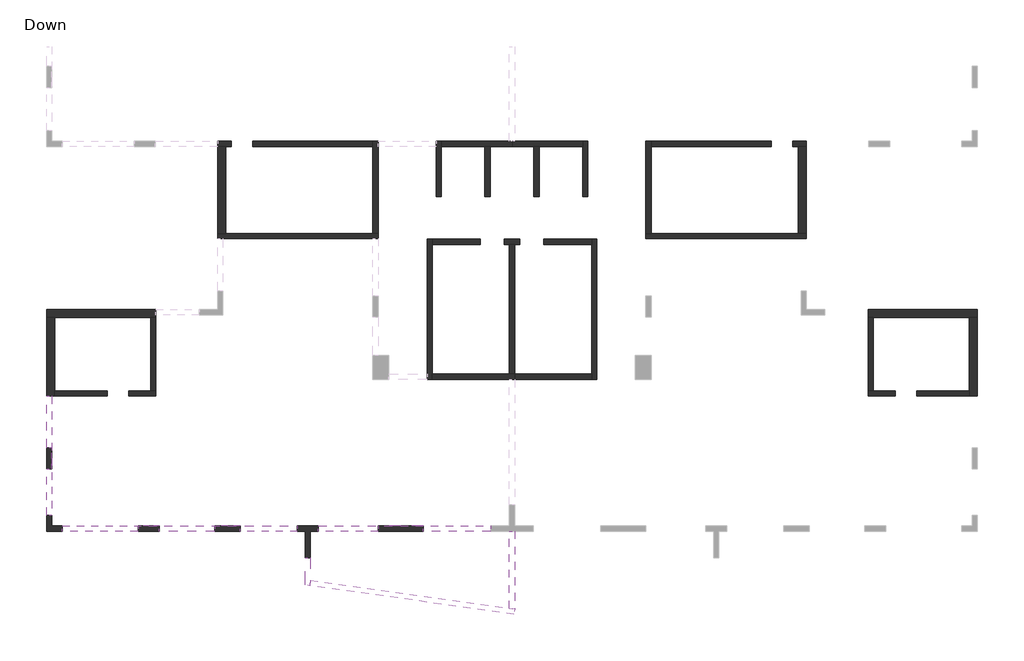
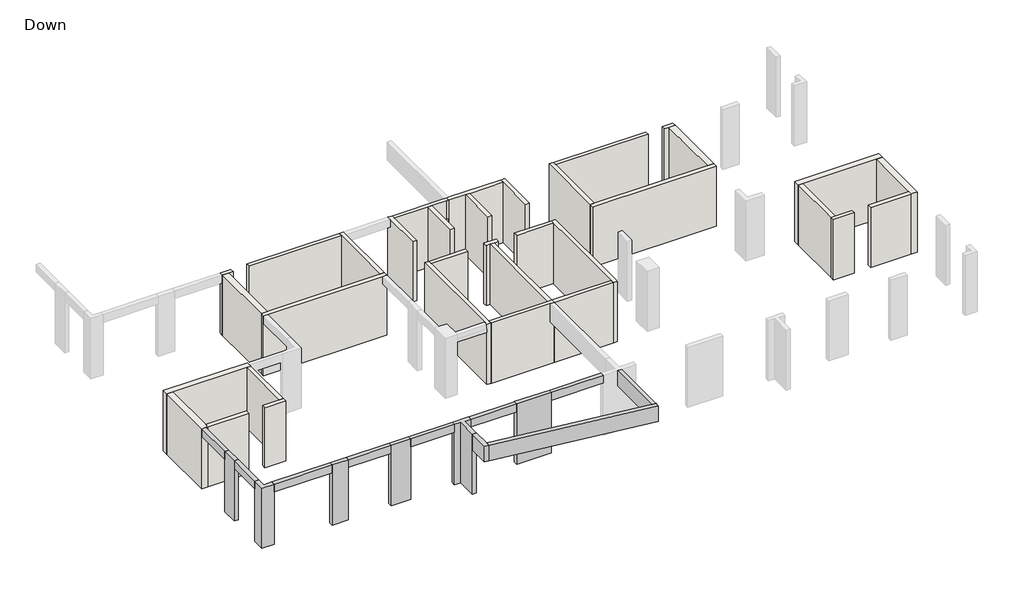
# One storey, part 1 of 2: 34 walls, 10 beams, 6 columns.
"""IFC4 building model written with IfcOpenShell, lengths in millimetres."""

from ifc_helpers import new_model, si_unit, origin, origin_with_axes, place, context, project, spatial, polyline, outline, extrude, faceted_brep, element, save

model = new_model("IFC4")

# Units and contexts
model_context = context("Model", 3, world=origin())
ifc_project = project(units=[si_unit("LENGTHUNIT", "METRE", prefix="MILLI")], contexts=[model_context])

# Site, building, storey
site = spatial("IfcSite", under=ifc_project)
building = spatial("IfcBuilding", under=site)
storey = spatial("IfcBuildingStorey", under=building, Name="Down", Elevation=0.0)

# Beams
placement = place(None, origin())
element("IfcBeam", 1, ObjectType="Concrete Rectengular Beam : 20/40", at=placement, inside=storey, context=model_context, shape_type="Brep", body=[
    faceted_brep([(-5966.3203921, -13204.5252202, 3120.0), (-3416.392751, -13204.5252202, 3120.0), (-3416.392751, -13009.5252202, 3120.0), (-5966.3203921, -13009.5252202, 3120.0), (-3416.392751, -13004.5252202, 2720.0), (-6816.392751, -13004.5252202, 2720.0), (-6816.392751, -13004.5252202, 2890.0), (-3416.392751, -13004.5252202, 2890.0), (-3416.392751, -13204.5252202, 2720.0), (-5966.3203921, -13204.5252202, 2720.0), (-5966.3203921, -13005.5744243, 2720.0), (-6816.392751, -13005.5744243, 2720.0), (-5966.3203921, -13204.5252202, 2890.0), (-6816.392751, -13005.5744243, 2890.0), (-3416.392751, -13009.5252202, 2890.0), (-5966.3203921, -13005.5744243, 2890.0), (-5966.3203921, -13009.5252202, 2890.0)], [[[0, 1, 2, 3]], [[4, 5, 6, 7]], [[5, 4, 8, 9, 10, 11]], [[8, 1, 0, 12, 9]], [[5, 11, 13, 6]], [[8, 4, 7, 14, 2, 1]], [[11, 10, 15, 13]], [[10, 9, 12, 0, 3, 16, 15]], [[16, 14, 7, 6, 13, 15]], [[14, 16, 3, 2]]]),
])
element("IfcBeam", 2, ObjectType="Concrete Rectengular Beam : 20/40", at=placement, inside=storey, context=model_context, shape_type="Brep", body=[
    faceted_brep([(-7666.3203921, -13204.5252202, 3120.0), (-7666.3203921, -13009.5252202, 3120.0), (-9916.193764, -13009.5252202, 3120.0), (-9916.193764, -13204.5252202, 3120.0), (-6816.392751, -13004.5252202, 2890.0), (-6816.392751, -13004.5252202, 2720.0), (-9916.193764, -13004.5252202, 2720.0), (-9916.193764, -13004.5252202, 2890.0), (-6816.392751, -13005.5744243, 2720.0), (-7666.3203921, -13005.5744243, 2720.0), (-7666.3203921, -13204.5252202, 2720.0), (-9916.193764, -13204.5252202, 2720.0), (-7666.3203921, -13204.5252202, 2890.0), (-6816.392751, -13005.5744243, 2890.0), (-7666.3203921, -13005.5744243, 2890.0), (-7666.3203921, -13009.5252202, 2890.0), (-9916.193764, -13009.5252202, 2890.0)], [[[0, 1, 2, 3]], [[4, 5, 6, 7]], [[5, 8, 9, 10, 11, 6]], [[10, 12, 0, 3, 11]], [[8, 5, 4, 13]], [[9, 8, 13, 14]], [[10, 9, 14, 15, 1, 0, 12]], [[13, 4, 7, 16, 15, 14]], [[1, 15, 16, 2]], [[3, 2, 16, 7, 6, 11]]]),
])
element("IfcBeam", 3, ObjectType="Concrete Rectengular Beam : 20/40", at=placement, inside=storey, context=model_context, shape_type="Brep", body=[
    faceted_brep([(-12866.5555585, -13009.5252202, 3120.0), (-12866.5555585, -13204.5252202, 3120.0), (-10716.193764, -13204.5252202, 3120.0), (-10716.193764, -13009.5252202, 3120.0), (-13341.5555585, -13004.5252202, 2720.0), (-13341.5555585, -13004.5252202, 2890.0), (-10716.193764, -13004.5252202, 2890.0), (-10716.193764, -13004.5252202, 2720.0), (-13341.5555585, -13005.8747137, 2720.0), (-10716.193764, -13204.5252202, 2720.0), (-12866.5555585, -13204.5252202, 2720.0), (-12866.5555585, -13005.8747137, 2720.0), (-13341.5555585, -13005.8747137, 2890.0), (-12866.5555585, -13005.8747137, 2890.0), (-12866.5555585, -13009.5252202, 2890.0), (-10716.193764, -13009.5252202, 2890.0)], [[[0, 1, 2, 3]], [[4, 5, 6, 7]], [[8, 4, 7, 9, 10, 11]], [[1, 10, 9, 2]], [[4, 8, 12, 5]], [[8, 11, 13, 12]], [[11, 10, 1, 0, 14, 13]], [[5, 12, 13, 14, 15, 6]], [[14, 0, 3, 15]], [[3, 2, 9, 7, 6, 15]]]),
])
element("IfcBeam", 4, ObjectType="Concrete Rectengular Beam : 20/40", at=placement, inside=storey, context=model_context, shape_type="Brep", body=[
    faceted_brep([(-15916.4289304, -13204.5252202, 3120.0), (-13816.5555585, -13204.5252202, 3120.0), (-13816.5555585, -13009.5252202, 3120.0), (-15916.4289304, -13009.5252202, 3120.0), (-13341.5555585, -13004.5252202, 2720.0), (-16316.4289304, -13004.5252202, 2720.0), (-16316.4289304, -13004.5252202, 2890.0), (-13341.5555585, -13004.5252202, 2890.0), (-13341.5555585, -13005.8747137, 2720.0), (-13816.5555585, -13005.8747137, 2720.0), (-13816.5555585, -13204.5252202, 2720.0), (-15916.4289304, -13204.5252202, 2720.0), (-15916.4289304, -13005.8747137, 2720.0), (-16316.4289304, -13005.8747137, 2720.0), (-16316.4289304, -13005.8747137, 2890.0), (-13341.5555585, -13005.8747137, 2890.0), (-15916.4289304, -13005.8747137, 2890.0), (-15916.4289304, -13009.5252202, 2890.0), (-13816.5555585, -13005.8747137, 2890.0), (-13816.5555585, -13009.5252202, 2890.0)], [[[0, 1, 2, 3]], [[4, 5, 6, 7]], [[5, 4, 8, 9, 10, 11, 12, 13]], [[0, 11, 10, 1]], [[5, 13, 14, 6]], [[8, 4, 7, 15]], [[13, 12, 16, 14]], [[12, 11, 0, 3, 17, 16]], [[9, 8, 15, 18]], [[10, 9, 18, 19, 2, 1]], [[17, 19, 18, 15, 7, 6, 14, 16]], [[19, 17, 3, 2]]]),
])
element("IfcBeam", 5, ObjectType="Concrete Rectengular Beam : 20/40", at=placement, inside=storey, context=model_context, shape_type="Brep", body=[
    faceted_brep([(-19564.2400737, -13204.5252202, 3120.0), (-16716.4289304, -13204.5252202, 3120.0), (-16716.4289304, -13009.5252202, 3120.0), (-19564.2400737, -13009.5252202, 3120.0), (-16316.4289304, -13004.5252202, 2720.0), (-19564.2400737, -13004.5252202, 2720.0), (-19564.2400737, -13004.5252202, 2890.0), (-16316.4289304, -13004.5252202, 2890.0), (-16316.4289304, -13005.8747137, 2720.0), (-16716.4289304, -13005.8747137, 2720.0), (-16716.4289304, -13204.5252202, 2720.0), (-19564.2400737, -13204.5252202, 2720.0), (-16316.4289304, -13005.8747137, 2890.0), (-19564.2400737, -13009.5252202, 2890.0), (-16716.4289304, -13005.8747137, 2890.0), (-16716.4289304, -13009.5252202, 2890.0)], [[[0, 1, 2, 3]], [[4, 5, 6, 7]], [[5, 4, 8, 9, 10, 11]], [[0, 11, 10, 1]], [[8, 4, 7, 12]], [[5, 11, 0, 3, 13, 6]], [[9, 8, 12, 14]], [[10, 9, 14, 15, 2, 1]], [[13, 15, 14, 12, 7, 6]], [[15, 13, 3, 2]]]),
])
element("IfcBeam", 6, ObjectType="Concrete Rectengular Beam : 20/40", at=placement, inside=storey, context=model_context, shape_type="Brep", body=[
    faceted_brep([(-20164.2400737, -10855.1764503, 3120.0), (-20164.2400737, -12604.5252202, 3120.0), (-19966.2400737, -12604.5252202, 3120.0), (-19966.2400737, -10855.1764503, 3120.0), (-19964.2400737, -12604.5252202, 2720.0), (-19964.2400737, -10455.1764503, 2720.0), (-19964.2400737, -10455.1764503, 2890.0), (-19964.2400737, -12604.5252202, 2890.0), (-20164.2400737, -12604.5252202, 2720.0), (-20164.2400737, -10855.1764503, 2720.0), (-19965.2892778, -10855.1764503, 2720.0), (-19965.2892778, -10455.1764503, 2720.0), (-19965.2892778, -10455.1764503, 2890.0), (-19966.2400737, -12604.5252202, 2890.0), (-19965.2892778, -10855.1764503, 2890.0), (-19966.2400737, -10855.1764503, 2890.0)], [[[0, 1, 2, 3]], [[4, 5, 6, 7]], [[5, 4, 8, 9, 10, 11]], [[8, 1, 0, 9]], [[5, 11, 12, 6]], [[8, 4, 7, 13, 2, 1]], [[11, 10, 14, 12]], [[10, 9, 0, 3, 15, 14]], [[15, 13, 7, 6, 12, 14]], [[13, 15, 3, 2]]]),
])
element("IfcBeam", 7, ObjectType="Concrete Rectengular Beam : 20/40", at=placement, inside=storey, context=model_context, shape_type="Brep", body=[
    faceted_brep([(-20164.2400737, -8105.8819496, 3120.0), (-20164.2400737, -10055.1764503, 3120.0), (-19966.2400737, -10055.1764503, 3120.0), (-19966.2400737, -8105.8819496, 3120.0), (-19964.2400737, -10455.1764503, 2720.0), (-19964.2400737, -8105.8819496, 2720.0), (-19964.2400737, -8105.8819496, 2890.0), (-19964.2400737, -10455.1764503, 2890.0), (-19965.2892778, -10455.1764503, 2720.0), (-19965.2892778, -10055.1764503, 2720.0), (-20164.2400737, -10055.1764503, 2720.0), (-20164.2400737, -8105.8819496, 2720.0), (-19965.2892778, -10455.1764503, 2890.0), (-19965.2892778, -10055.1764503, 2890.0), (-19966.2400737, -10055.1764503, 2890.0), (-19966.2400737, -8105.8819496, 2890.0)], [[[0, 1, 2, 3]], [[4, 5, 6, 7]], [[4, 8, 9, 10, 11, 5]], [[10, 1, 0, 11]], [[8, 4, 7, 12]], [[9, 8, 12, 13]], [[10, 9, 13, 14, 2, 1]], [[5, 11, 0, 3, 15, 6]], [[15, 14, 13, 12, 7, 6]], [[14, 15, 3, 2]]]),
])
element("IfcBeam", 8, ObjectType="Concrete Rectengular Beam : 20/80", at=placement, inside=storey, context=model_context, shape_type="Brep", body=[
    faceted_brep([(-10416.193764, -15232.5030981, 3120.0), (-10216.193764, -15260.611265, 3120.0), (-10216.193764, -15058.6457505, 3120.0), (-10216.193764, -14204.5252202, 3120.0), (-10416.193764, -14204.5252202, 3120.0), (-10416.193764, -15232.5030981, 2320.0), (-10416.193764, -14204.5252202, 2320.0), (-10216.193764, -15260.611265, 2320.0), (-10216.193764, -14204.5252202, 2320.0), (-10216.193764, -15058.6457505, 2320.0)], [[[0, 1, 2, 3, 4]], [[5, 0, 4, 6]], [[7, 5, 6, 8, 9]], [[1, 7, 9, 8, 3, 2]], [[4, 3, 8, 6]], [[1, 0, 5, 7]]]),
])
element("IfcBeam", 9, ObjectType="Concrete Rectengular Beam : 20/80", at=placement, inside=storey, context=model_context, shape_type="Brep", body=[
    faceted_brep([(-10216.193764, -15058.6457505, 3120.0), (-10216.193764, -15260.611265, 3120.0), (-2544.2273712, -16338.8358257, 3120.0), (-2541.3191471, -16318.142736, 3120.0), (-2516.392751, -16140.7822119, 3120.0), (-2716.392751, -16112.674045, 3120.0), (-10216.193764, -15260.611265, 2320.0), (-2544.2273712, -16338.8358257, 2320.0), (-10216.193764, -15058.6457505, 2320.0), (-2716.392751, -16112.674045, 2320.0), (-2516.392751, -16140.7822119, 2320.0), (-2541.3191471, -16318.142736, 2320.0), (-10216.193764, -15058.6457505, 2890.0)], [[[0, 1, 2, 3, 4, 5]], [[1, 6, 7, 2]], [[6, 8, 9, 10, 11, 7]], [[4, 10, 9, 8, 12, 0, 5]], [[1, 0, 12, 8, 6]], [[4, 3, 2, 7, 11, 10]]]),
])
element("IfcBeam", 10, ObjectType="Concrete Rectengular Beam : 20/80", at=placement, inside=storey, context=model_context, shape_type="Brep", body=[
    faceted_brep([(-2516.392751, -13204.5252202, 3120.0), (-2716.392751, -13204.5252202, 3120.0), (-2716.392751, -16112.674045, 3120.0), (-2516.392751, -16140.7822119, 3120.0), (-2516.392751, -16112.674045, 3120.0), (-2516.392751, -13204.5252202, 2320.0), (-2516.392751, -13204.5252202, 2890.0), (-2516.392751, -16140.7822119, 2320.0), (-2516.392751, -16112.674045, 2320.0), (-2716.392751, -13204.5252202, 2320.0), (-2716.392751, -16112.674045, 2320.0), (-2716.392751, -13204.5252202, 2890.0), (-2716.392751, -16112.674045, 2890.0)], [[[0, 1, 2, 3, 4]], [[5, 6, 0, 4, 3, 7, 8]], [[9, 5, 8, 7, 10]], [[1, 11, 9, 10, 12, 2]], [[1, 0, 6, 5, 9, 11]], [[3, 2, 12, 10, 7]]]),
])

# Columns
element("IfcColumn", 11, ObjectType="Concrete Rectengular Column : 170/20", at=placement, inside=storey, context=model_context, shape_type="Brep", body=[
    faceted_brep([(-7666.3203921, -13005.5744243, 0.0), (-5966.3203921, -13005.5744243, 0.0), (-5966.3203921, -13205.5744243, 0.0), (-7666.3203921, -13205.5744243, 0.0), (-7666.3203921, -13005.5744243, 3120.0), (-5966.3203921, -13005.5744243, 3120.0), (-5966.3203921, -13005.5744243, 2890.0), (-7666.3203921, -13005.5744243, 2890.0), (-5966.3203921, -13009.5252202, 3120.0), (-5966.3203921, -13204.5252202, 3120.0), (-5966.3203921, -13205.5744243, 3120.0), (-5966.3203921, -13205.5744243, 2890.0), (-7666.3203921, -13205.5744243, 3120.0), (-7666.3203921, -13205.5744243, 2890.0), (-7666.3203921, -13204.5252202, 3120.0), (-7666.3203921, -13009.5252202, 3120.0)], [[[0, 1, 2, 3]], [[4, 5, 6, 1, 0, 7]], [[5, 8, 9, 10, 11, 2, 1, 6]], [[10, 12, 13, 3, 2, 11]], [[12, 14, 15, 4, 7, 0, 3, 13]], [[4, 15, 14, 12, 10, 9, 8, 5]]]),
])
element("IfcColumn", 12, ObjectType="Concrete Rectengular Column : 80/20", at=placement, inside=storey, context=model_context, shape_type="Brep", body=[
    faceted_brep([(-16716.4289304, -13005.8747137, 0.0), (-15916.4289304, -13005.8747137, 0.0), (-15916.4289304, -13205.8747137, 0.0), (-16716.4289304, -13205.8747137, 0.0), (-16716.4289304, -13005.8747137, 3120.0), (-15916.4289304, -13005.8747137, 3120.0), (-15916.4289304, -13005.8747137, 2890.0), (-16716.4289304, -13005.8747137, 2890.0), (-15916.4289304, -13009.5252202, 3120.0), (-15916.4289304, -13205.8747137, 3120.0), (-16716.4289304, -13205.8747137, 3120.0), (-16716.4289304, -13009.5252202, 3120.0)], [[[0, 1, 2, 3]], [[4, 5, 6, 1, 0, 7]], [[5, 8, 9, 2, 1, 6]], [[9, 10, 3, 2]], [[10, 11, 4, 7, 0, 3]], [[4, 11, 10, 9, 8, 5]]]),
])
element("IfcColumn", 13, ObjectType="Concrete Rectengular Column : 80/20", at=placement, inside=storey, context=model_context, shape_type="Brep", body=[
    faceted_brep([(-19965.2892778, -10055.1764503, 0.0), (-19965.2892778, -10855.1764503, 0.0), (-20165.2892778, -10855.1764503, 0.0), (-20165.2892778, -10055.1764503, 0.0), (-19965.2892778, -10055.1764503, 3120.0), (-19965.2892778, -10855.1764503, 3120.0), (-19965.2892778, -10855.1764503, 2890.0), (-19965.2892778, -10055.1764503, 2890.0), (-19966.2400737, -10855.1764503, 3120.0), (-20165.2892778, -10855.1764503, 3120.0), (-20165.2892778, -10055.1764503, 3120.0), (-19966.2400737, -10055.1764503, 3120.0)], [[[0, 1, 2, 3]], [[4, 5, 6, 1, 0, 7]], [[5, 8, 9, 2, 1, 6]], [[9, 10, 3, 2]], [[10, 11, 4, 7, 0, 3]], [[4, 11, 10, 9, 8, 5]]]),
])
element("IfcColumn", 14, ObjectType="Concrete Rectengular Column : 95/20", at=placement, inside=storey, context=model_context, shape_type="Brep", body=[
    faceted_brep([(-13816.5555585, -13005.8747137, 0.0), (-12866.5555585, -13005.8747137, 0.0), (-12866.5555585, -13205.8747137, 0.0), (-13816.5555585, -13205.8747137, 0.0), (-13816.5555585, -13005.8747137, 3120.0), (-12866.5555585, -13005.8747137, 3120.0), (-12866.5555585, -13005.8747137, 2890.0), (-13816.5555585, -13005.8747137, 2890.0), (-12866.5555585, -13009.5252202, 3120.0), (-12866.5555585, -13205.8747137, 3120.0), (-13816.5555585, -13205.8747137, 3120.0), (-13816.5555585, -13009.5252202, 3120.0)], [[[0, 1, 2, 3]], [[4, 5, 6, 1, 0, 7]], [[5, 8, 9, 2, 1, 6]], [[9, 10, 3, 2]], [[10, 11, 4, 7, 0, 3]], [[4, 11, 10, 9, 8, 5]]]),
])
element("IfcColumn", 15, ObjectType="L Column : 60/60/20/20", at=placement, inside=storey, context=model_context, shape_type="Brep", body=[
    faceted_brep([(-20164.2400737, -13204.5252202, 0.0), (-20164.2400737, -12604.5252202, 0.0), (-19964.2400737, -12604.5252202, 0.0), (-19964.2400737, -13004.5252202, 0.0), (-19564.2400737, -13004.5252202, 0.0), (-19564.2400737, -13204.5252202, 0.0), (-20164.2400737, -13204.5252202, 3120.0), (-20164.2400737, -12604.5252202, 3120.0), (-19966.2400737, -12604.5252202, 3120.0), (-19964.2400737, -12604.5252202, 3120.0), (-19964.2400737, -12604.5252202, 2890.0), (-19964.2400737, -13004.5252202, 3120.0), (-19964.2400737, -13004.5252202, 2890.0), (-19564.2400737, -13004.5252202, 3120.0), (-19564.2400737, -13004.5252202, 2890.0), (-19564.2400737, -13009.5252202, 3120.0), (-19564.2400737, -13204.5252202, 3120.0)], [[[0, 1, 2, 3, 4, 5]], [[6, 7, 1, 0]], [[7, 8, 9, 10, 2, 1]], [[9, 11, 12, 3, 2, 10]], [[11, 13, 14, 4, 3, 12]], [[13, 15, 16, 5, 4, 14]], [[16, 6, 0, 5]], [[6, 16, 15, 13, 11, 9, 8, 7]]]),
])
element("IfcColumn", 16, ObjectType="T Column : 120/80/20/20", at=placement, inside=storey, context=model_context, shape_type="Brep", body=[
    faceted_brep([(-10416.193764, -14204.5252202, 0.0), (-10416.193764, -13204.5252202, 0.0), (-10716.193764, -13204.5252202, 0.0), (-10716.193764, -13004.5252202, 0.0), (-9916.193764, -13004.5252202, 0.0), (-9916.193764, -13204.5252202, 0.0), (-10216.193764, -13204.5252202, 0.0), (-10216.193764, -14204.5252202, 0.0), (-10416.193764, -14204.5252202, 3120.0), (-10416.193764, -13204.5252202, 3120.0), (-10716.193764, -13204.5252202, 3120.0), (-10716.193764, -13009.5252202, 3120.0), (-10716.193764, -13004.5252202, 3120.0), (-10716.193764, -13004.5252202, 2890.0), (-9916.193764, -13004.5252202, 3120.0), (-9916.193764, -13004.5252202, 2890.0), (-9916.193764, -13009.5252202, 3120.0), (-9916.193764, -13204.5252202, 3120.0), (-10216.193764, -13204.5252202, 3120.0), (-10216.193764, -13204.5252202, 2890.0), (-10216.193764, -14204.5252202, 3120.0)], [[[0, 1, 2, 3, 4, 5, 6, 7]], [[8, 9, 1, 0]], [[9, 10, 2, 1]], [[10, 11, 12, 13, 3, 2]], [[12, 14, 15, 4, 3, 13]], [[14, 16, 17, 5, 4, 15]], [[17, 18, 19, 6, 5]], [[18, 20, 7, 6, 19]], [[20, 8, 0, 7]], [[8, 20, 18, 17, 16, 14, 12, 11, 10, 9]]]),
])

# Walls
element("IfcWall", 17, ObjectType="20", at=placement, inside=storey, context=model_context, shape_type="Brep", body=[
    faceted_brep([(-13715.271188, -2169.1055386, 0.0), (-7666.3203921, -2169.1055386, 0.0), (-7666.3203921, -2169.1055386, 3120.0), (-7866.3203921, -2169.1055386, 3120.0), (-13515.271188, -2169.1055386, 3120.0), (-13715.271188, -2169.1055386, 3120.0), (-13715.271188, -2169.1055386, 2720.0), (-13715.271188, -1969.1055386, 0.0), (-13715.271188, -1969.1055386, 3120.0), (-13415.271188, -1969.1055386, 3120.0), (-7866.3203921, -1969.1055386, 3120.0), (-7666.3203921, -1969.1055386, 3120.0), (-7666.3203921, -1969.1055386, 0.0), (-7866.3203921, -1969.1055386, 0.0), (-13415.271188, -1969.1055386, 0.0)], [[[0, 1, 2, 3, 4, 5, 6]], [[7, 8, 9, 10, 11, 12, 13, 14]], [[1, 0, 7, 14, 13, 12]], [[5, 4, 3, 2, 11, 10, 9, 8]], [[2, 1, 12, 11]], [[0, 6, 5, 8, 7]]]),
])
element("IfcWall", 18, ObjectType="20", at=placement, inside=storey, context=model_context, shape_type="Brep", body=[
    faceted_brep([(-7666.3203921, -1969.1055386, 0.0), (-7666.3203921, 1513.6006842, 0.0), (-7666.3203921, 1513.6006842, 2720.0), (-7666.3203921, 1513.6006842, 3120.0), (-7666.3203921, 1313.6006842, 3120.0), (-7666.3203921, -1969.1055386, 3120.0), (-7866.3203921, -1969.1055386, 0.0), (-7866.3203921, -1969.1055386, 2890.0), (-7866.3203921, -1969.1055386, 3120.0), (-7866.3203921, 1313.6006842, 3120.0), (-7866.3203921, 1513.6006842, 3120.0), (-7866.3203921, 1513.6006842, 0.0), (-7866.3203921, 1313.6006842, 0.0)], [[[0, 1, 2, 3, 4, 5]], [[6, 7, 8, 9, 10, 11, 12]], [[1, 0, 6, 12, 11]], [[5, 4, 3, 10, 9, 8]], [[0, 5, 8, 7, 6]], [[3, 2, 1, 11, 10]]]),
])
element("IfcWall", 19, ObjectType="20", at=placement, inside=storey, context=model_context, shape_type="Brep", body=[
    faceted_brep([(-7866.3203921, 1513.6006842, 0.0), (-12396.6930404, 1513.6006842, 0.0), (-12396.6930404, 1513.6006842, 2890.0), (-12396.6930404, 1513.6006842, 3120.0), (-7866.3203921, 1513.6006842, 3120.0), (-7866.3203921, 1313.6006842, 0.0), (-7866.3203921, 1313.6006842, 2890.0), (-7866.3203921, 1313.6006842, 3120.0), (-12396.6930404, 1313.6006842, 3120.0), (-12396.6930404, 1313.6006842, 2890.0), (-12396.6930404, 1313.6006842, 0.0), (-12396.6930404, 1413.6006842, 3120.0)], [[[0, 1, 2, 3, 4]], [[5, 6, 7, 8, 9, 10]], [[1, 0, 5, 10]], [[3, 2, 1, 10, 9, 8, 11]], [[4, 3, 11, 8, 7]], [[0, 4, 7, 6, 5]]]),
])
element("IfcWall", 20, ObjectType="20", at=placement, inside=storey, context=model_context, shape_type="Brep", body=[
    faceted_brep([(-13196.7292199, 1514.1252863, 0.0), (-13715.271188, 1514.1252863, 0.0), (-13715.271188, 1514.1252863, 2720.0), (-13715.271188, 1514.1252863, 3120.0), (-13196.7292199, 1514.1252863, 3120.0), (-13196.7292199, 1514.1252863, 2890.0), (-13196.7292199, 1314.1252863, 0.0), (-13196.7292199, 1314.1252863, 3120.0), (-13415.271188, 1314.1252863, 3120.0), (-13715.271188, 1314.1252863, 3120.0), (-13715.271188, 1314.1252863, 2720.0), (-13715.271188, 1314.1252863, 0.0), (-13415.271188, 1314.1252863, 0.0), (-13196.7292199, 1413.6006842, 3120.0)], [[[0, 1, 2, 3, 4, 5]], [[6, 7, 8, 9, 10, 11, 12]], [[1, 0, 6, 12, 11]], [[4, 3, 9, 8, 7, 13]], [[0, 5, 4, 13, 7, 6]], [[3, 2, 1, 11, 10, 9]]]),
])
element("IfcWall", 21, ObjectType="20", at=placement, inside=storey, context=model_context, shape_type="Brep", body=[
    faceted_brep([(-19864.2400737, -8104.8146558, 0.0), (-17867.839929, -8104.8146558, 0.0), (-17867.839929, -8104.8146558, 2890.0), (-17867.839929, -8104.8146558, 3120.0), (-19864.2400737, -8104.8146558, 3120.0), (-19864.2400737, -8104.8146558, 2890.0), (-19864.2400737, -7904.8146558, 0.0), (-19864.2400737, -7904.8146558, 2890.0), (-19864.2400737, -7904.8146558, 3120.0), (-17867.839929, -7904.8146558, 3120.0), (-17867.839929, -7904.8146558, 2890.0), (-17867.839929, -7904.8146558, 0.0), (-17867.839929, -8004.8146558, 3120.0)], [[[0, 1, 2, 3, 4, 5]], [[6, 7, 8, 9, 10, 11]], [[1, 0, 6, 11]], [[3, 2, 1, 11, 10, 9, 12]], [[4, 3, 12, 9, 8]], [[0, 5, 4, 8, 7, 6]]]),
])
element("IfcWall", 22, ObjectType="20", at=placement, inside=storey, context=model_context, shape_type="Brep", body=[
    faceted_brep([(-17067.8037495, -8104.8146558, 0.0), (-16045.535298, -8104.8146558, 0.0), (-16045.535298, -8104.8146558, 2890.0), (-16045.535298, -8104.8146558, 3120.0), (-17067.8037495, -8104.8146558, 3120.0), (-17067.8037495, -8104.8146558, 2890.0), (-17067.8037495, -7904.8146558, 0.0), (-17067.8037495, -7904.8146558, 2890.0), (-17067.8037495, -7904.8146558, 3120.0), (-16245.535298, -7904.8146558, 3120.0), (-16045.535298, -7904.8146558, 3120.0), (-16045.535298, -7904.8146558, 0.0), (-16245.535298, -7904.8146558, 0.0), (-17067.8037495, -8004.8146558, 3120.0)], [[[0, 1, 2, 3, 4, 5]], [[6, 7, 8, 9, 10, 11, 12]], [[1, 0, 6, 12, 11]], [[4, 3, 10, 9, 8, 13]], [[0, 5, 4, 13, 8, 7, 6]], [[3, 2, 1, 11, 10]]]),
])
element("IfcWall", 23, ObjectType="20", at=placement, inside=storey, context=model_context, shape_type="Brep", body=[
    faceted_brep([(-16045.535298, -7904.8146558, 0.0), (-16045.535298, -5135.8928035, 0.0), (-16045.535298, -5135.8928035, 3120.0), (-16045.535298, -7904.8146558, 3120.0), (-16245.535298, -7904.8146558, 0.0), (-16245.535298, -7904.8146558, 2890.0), (-16245.535298, -7904.8146558, 3120.0), (-16245.535298, -5135.8928035, 3120.0), (-16245.535298, -5135.8928035, 2890.0), (-16245.535298, -5135.8928035, 0.0)], [[[0, 1, 2, 3]], [[4, 5, 6, 7, 8, 9]], [[1, 0, 4, 9]], [[3, 2, 7, 6]], [[0, 3, 6, 5, 4]], [[2, 1, 9, 8, 7]]]),
])
element("IfcWall", 24, ObjectType="20", at=placement, inside=storey, context=model_context, shape_type="Brep", body=[
    faceted_brep([(-5816.5012893, -2183.9210234, 0.0), (-5816.5012893, -7475.1655965, 0.0), (-5816.5012893, -7475.1655965, 2720.0), (-5816.5012893, -7475.1655965, 2890.0), (-5816.5012893, -7475.1655965, 3120.0), (-5816.5012893, -7275.6540191, 3120.0), (-5816.5012893, -2183.9210234, 3120.0), (-5816.5012893, -2183.9210234, 2890.0), (-5616.5012893, -2183.9210234, 0.0), (-5616.5012893, -2183.9210234, 3120.0), (-5616.5012893, -2383.9210234, 3120.0), (-5616.5012893, -3585.0425864, 3120.0), (-5616.5012893, -7275.1655965, 3120.0), (-5616.5012893, -7475.1655965, 3120.0), (-5616.5012893, -7475.1655965, 0.0), (-5616.5012893, -7275.1655965, 0.0), (-5616.5012893, -2383.9210234, 0.0)], [[[0, 1, 2, 3, 4, 5, 6, 7]], [[8, 9, 10, 11, 12, 13, 14, 15, 16]], [[1, 0, 8, 16, 15, 14]], [[6, 5, 4, 13, 12, 11, 10, 9]], [[0, 7, 6, 9, 8]], [[4, 3, 2, 1, 14, 13]]]),
])
element("IfcWall", 25, ObjectType="20", at=placement, inside=storey, context=model_context, shape_type="Brep", body=[
    faceted_brep([(-5616.5012893, -2383.9210234, 0.0), (-3816.4108407, -2383.9210234, 0.0), (-3816.4108407, -2383.9210234, 2890.0), (-3816.4108407, -2383.9210234, 3120.0), (-5616.5012893, -2383.9210234, 3120.0), (-5616.5012893, -2383.9210234, 2890.0), (-5616.5012893, -2183.9210234, 0.0), (-5616.5012893, -2183.9210234, 3120.0), (-3816.4108407, -2183.9210234, 3120.0), (-3816.4108407, -2183.9210234, 2890.0), (-3816.4108407, -2183.9210234, 0.0), (-3816.4108407, -2283.9210234, 3120.0)], [[[0, 1, 2, 3, 4, 5]], [[6, 7, 8, 9, 10]], [[1, 0, 6, 10]], [[3, 2, 1, 10, 9, 8, 11]], [[4, 3, 11, 8, 7]], [[0, 5, 4, 7, 6]]]),
])
element("IfcWall", 26, ObjectType="20", at=placement, inside=storey, context=model_context, shape_type="Brep", body=[
    faceted_brep([(-5616.5012893, -7475.1655965, 0.0), (-2517.9484673, -7475.1655965, 0.0), (-2517.9484673, -7475.1655965, 3120.0), (-2716.392751, -7475.1655965, 3120.0), (-5616.5012893, -7475.1655965, 3120.0), (-5616.5012893, -7275.1655965, 0.0), (-5616.5012893, -7275.1655965, 3120.0), (-2717.9484673, -7275.1655965, 3120.0), (-2517.9484673, -7275.1655965, 3120.0), (-2517.9484673, -7275.1655965, 0.0), (-2717.9484673, -7275.1655965, 0.0)], [[[0, 1, 2, 3, 4]], [[5, 6, 7, 8, 9, 10]], [[1, 0, 5, 10, 9]], [[4, 3, 2, 8, 7, 6]], [[0, 4, 6, 5]], [[2, 1, 9, 8]]]),
])
element("IfcWall", 27, ObjectType="20", at=placement, inside=storey, context=model_context, shape_type="Brep", body=[
    faceted_brep([(-2717.9484673, -2383.9210234, 0.0), (-2717.9484673, -7275.1655965, 0.0), (-2717.9484673, -7275.1655965, 3120.0), (-2717.9484673, -3585.0425864, 3120.0), (-2717.9484673, -2383.9210234, 3120.0), (-2717.9484673, -2383.9210234, 2890.0), (-2517.9484673, -2383.9210234, 0.0), (-2517.9484673, -2383.9210234, 2890.0), (-2517.9484673, -2383.9210234, 3120.0), (-2517.9484673, -3585.0425864, 3120.0), (-2517.9484673, -7275.1655965, 3120.0), (-2517.9484673, -7275.1655965, 0.0)], [[[0, 1, 2, 3, 4, 5]], [[6, 7, 8, 9, 10, 11]], [[1, 0, 6, 11]], [[4, 3, 2, 10, 9, 8]], [[2, 1, 11, 10]], [[0, 5, 4, 8, 7, 6]]]),
])
element("IfcWall", 28, ObjectType="20", at=placement, inside=storey, context=model_context, shape_type="Brep", body=[
    faceted_brep([(-2916.8992633, -2383.9210234, 0.0), (-2717.9484673, -2383.9210234, 0.0), (-2517.9484673, -2383.9210234, 0.0), (-2315.8862387, -2383.9210234, 0.0), (-2315.8862387, -2383.9210234, 2890.0), (-2315.8862387, -2383.9210234, 3120.0), (-2517.9484673, -2383.9210234, 3120.0), (-2717.9484673, -2383.9210234, 3120.0), (-2916.8992633, -2383.9210234, 3120.0), (-2916.8992633, -2383.9210234, 2890.0), (-2916.8992633, -2183.9210234, 0.0), (-2916.8992633, -2183.9210234, 2890.0), (-2916.8992633, -2183.9210234, 3120.0), (-2315.8862387, -2183.9210234, 3120.0), (-2315.8862387, -2183.9210234, 2890.0), (-2315.8862387, -2183.9210234, 0.0), (-2315.8862387, -2283.9210234, 3120.0), (-2916.8992633, -2283.9210234, 3120.0)], [[[0, 1, 2, 3, 4, 5, 6, 7, 8, 9]], [[10, 11, 12, 13, 14, 15]], [[3, 2, 1, 0, 10, 15]], [[5, 4, 3, 15, 14, 13, 16]], [[8, 7, 6, 5, 16, 13, 12, 17]], [[0, 9, 8, 17, 12, 11, 10]]]),
])
element("IfcWall", 29, ObjectType="20", at=placement, inside=storey, context=model_context, shape_type="Brep", body=[
    faceted_brep([(-5279.9781345, -585.9651624, 0.0), (-5279.9781345, 1313.6006842, 0.0), (-5279.9781345, 1513.6006842, 0.0), (-5279.9781345, 1513.6006842, 3120.0), (-5279.9781345, 1313.6006842, 3120.0), (-5279.9781345, -585.9651624, 3120.0), (-5479.9781345, -585.9651624, 0.0), (-5479.9781345, -585.9651624, 2890.0), (-5479.9781345, -585.9651624, 3120.0), (-5479.9781345, 1313.6006842, 3120.0), (-5479.9781345, 1513.6006842, 3120.0), (-5479.9781345, 1513.6006842, 2720.0), (-5479.9781345, 1513.6006842, 0.0)], [[[0, 1, 2, 3, 4, 5]], [[6, 7, 8, 9, 10, 11, 12]], [[2, 1, 0, 6, 12]], [[5, 4, 3, 10, 9, 8]], [[0, 5, 8, 7, 6]], [[3, 2, 12, 11, 10]]]),
])
element("IfcWall", 30, ObjectType="20", at=placement, inside=storey, context=model_context, shape_type="Brep", body=[
    faceted_brep([(-5279.9781345, 1313.6006842, 0.0), (-3638.6250231, 1313.6006842, 0.0), (-3438.6250231, 1313.6006842, 0.0), (-2616.3565715, 1313.6006842, 0.0), (-2616.3565715, 1313.6006842, 3120.0), (-3438.6250231, 1313.6006842, 3120.0), (-3638.6250231, 1313.6006842, 3120.0), (-5279.9781345, 1313.6006842, 3120.0), (-5279.9781345, 1513.6006842, 0.0), (-5279.9781345, 1513.6006842, 3120.0), (-2716.392751, 1513.6006842, 3120.0), (-2616.3565715, 1513.6006842, 3120.0), (-2616.3565715, 1513.6006842, 0.0)], [[[0, 1, 2, 3, 4, 5, 6, 7]], [[8, 9, 10, 11, 12]], [[3, 2, 1, 0, 8, 12]], [[4, 3, 12, 11]], [[7, 6, 5, 4, 11, 10, 9]], [[0, 7, 9, 8]]]),
])
element("IfcWall", 31, ObjectType="20", at=placement, inside=storey, context=model_context, shape_type="SweptSolid", body=[
    extrude(outline(polyline([(-3638.6250231, -585.9651624), (-3638.6250231, 1313.6006842), (-3438.6250231, 1313.6006842), (-3438.6250231, -585.9651624), (-3638.6250231, -585.9651624)])), origin_with_axes(), (0.0, 0.0, 1.0), 3120.0),
])
element("IfcWall", 32, ObjectType="20", at=placement, inside=storey, context=model_context, shape_type="Brep", body=[
    faceted_brep([(8482.4856861, -1969.1055386, 0.0), (8182.4856861, -1969.1055386, 0.0), (2633.5348901, -1969.1055386, 0.0), (2433.5348901, -1969.1055386, 0.0), (2433.5348901, -1969.1055386, 3120.0), (2633.5348901, -1969.1055386, 3120.0), (8182.4856861, -1969.1055386, 3120.0), (8482.4856861, -1969.1055386, 3120.0), (8482.4856861, -2169.1055386, 0.0), (8482.4856861, -2169.1055386, 2720.0), (8482.4856861, -2169.1055386, 3120.0), (8282.4856861, -2169.1055386, 3120.0), (2633.5348901, -2169.1055386, 3120.0), (2433.5348901, -2169.1055386, 3120.0), (2433.5348901, -2169.1055386, 0.0)], [[[0, 1, 2, 3, 4, 5, 6, 7]], [[8, 9, 10, 11, 12, 13, 14]], [[3, 2, 1, 0, 8, 14]], [[7, 6, 5, 4, 13, 12, 11, 10]], [[4, 3, 14, 13]], [[0, 7, 10, 9, 8]]]),
])
element("IfcWall", 33, ObjectType="20", at=placement, inside=storey, context=model_context, shape_type="Brep", body=[
    faceted_brep([(2633.5348901, -1969.1055386, 0.0), (2633.5348901, 1313.6006842, 0.0), (2633.5348901, 1513.6006842, 0.0), (2633.5348901, 1513.6006842, 3120.0), (2633.5348901, 1313.6006842, 3120.0), (2633.5348901, -1969.1055386, 3120.0), (2633.5348901, -1969.1055386, 2890.0), (2433.5348901, -1969.1055386, 0.0), (2433.5348901, -1969.1055386, 3120.0), (2433.5348901, 1313.6006842, 3120.0), (2433.5348901, 1513.6006842, 3120.0), (2433.5348901, 1513.6006842, 2720.0), (2433.5348901, 1513.6006842, 0.0)], [[[0, 1, 2, 3, 4, 5, 6]], [[7, 8, 9, 10, 11, 12]], [[2, 1, 0, 7, 12]], [[5, 4, 3, 10, 9, 8]], [[0, 6, 5, 8, 7]], [[3, 2, 12, 11, 10]]]),
])
element("IfcWall", 34, ObjectType="20", at=placement, inside=storey, context=model_context, shape_type="Brep", body=[
    faceted_brep([(2633.5348901, 1313.6006842, 0.0), (7163.9075385, 1313.6006842, 0.0), (7163.9075385, 1313.6006842, 2890.0), (7163.9075385, 1313.6006842, 3120.0), (2633.5348901, 1313.6006842, 3120.0), (2633.5348901, 1313.6006842, 2890.0), (2633.5348901, 1513.6006842, 0.0), (2633.5348901, 1513.6006842, 3120.0), (7163.9075385, 1513.6006842, 3120.0), (7163.9075385, 1513.6006842, 2890.0), (7163.9075385, 1513.6006842, 0.0), (7163.9075385, 1413.6006842, 3120.0)], [[[0, 1, 2, 3, 4, 5]], [[6, 7, 8, 9, 10]], [[1, 0, 6, 10]], [[3, 2, 1, 10, 9, 8, 11]], [[4, 3, 11, 8, 7]], [[0, 5, 4, 7, 6]]]),
])
element("IfcWall", 35, ObjectType="20", at=placement, inside=storey, context=model_context, shape_type="Brep", body=[
    faceted_brep([(7963.9437179, 1314.1252863, 0.0), (8182.4856861, 1314.1252863, 0.0), (8482.4856861, 1314.1252863, 0.0), (8482.4856861, 1314.1252863, 2720.0), (8482.4856861, 1314.1252863, 3120.0), (8182.4856861, 1314.1252863, 3120.0), (7963.9437179, 1314.1252863, 3120.0), (7963.9437179, 1514.1252863, 0.0), (7963.9437179, 1514.1252863, 2890.0), (7963.9437179, 1514.1252863, 3120.0), (8482.4856861, 1514.1252863, 3120.0), (8482.4856861, 1514.1252863, 2720.0), (8482.4856861, 1514.1252863, 0.0), (7963.9437179, 1413.6006842, 3120.0)], [[[0, 1, 2, 3, 4, 5, 6]], [[7, 8, 9, 10, 11, 12]], [[2, 1, 0, 7, 12]], [[6, 5, 4, 10, 9, 13]], [[0, 6, 13, 9, 8, 7]], [[4, 3, 2, 12, 11, 10]]]),
])
element("IfcWall", 36, ObjectType="20", at=placement, inside=storey, context=model_context, shape_type="Brep", body=[
    faceted_brep([(14631.4545717, -7904.8146558, 0.0), (12635.054427, -7904.8146558, 0.0), (12635.054427, -7904.8146558, 2890.0), (12635.054427, -7904.8146558, 3120.0), (14631.4545717, -7904.8146558, 3120.0), (14631.4545717, -7904.8146558, 2890.0), (14631.4545717, -8104.8146558, 0.0), (14631.4545717, -8104.8146558, 2890.0), (14631.4545717, -8104.8146558, 3120.0), (12635.054427, -8104.8146558, 3120.0), (12635.054427, -8104.8146558, 2890.0), (12635.054427, -8104.8146558, 0.0), (12635.054427, -8004.8146558, 3120.0)], [[[0, 1, 2, 3, 4, 5]], [[6, 7, 8, 9, 10, 11]], [[1, 0, 6, 11]], [[3, 2, 1, 11, 10, 9, 12]], [[4, 3, 12, 9, 8]], [[0, 5, 4, 8, 7, 6]]]),
])
element("IfcWall", 37, ObjectType="20", at=placement, inside=storey, context=model_context, shape_type="Brep", body=[
    faceted_brep([(11835.0182476, -7904.8146558, 0.0), (11012.749796, -7904.8146558, 0.0), (10812.749796, -7904.8146558, 0.0), (10812.749796, -7904.8146558, 3120.0), (11012.749796, -7904.8146558, 3120.0), (11835.0182476, -7904.8146558, 3120.0), (11835.0182476, -7904.8146558, 2890.0), (11835.0182476, -8104.8146558, 0.0), (11835.0182476, -8104.8146558, 2890.0), (11835.0182476, -8104.8146558, 3120.0), (10812.749796, -8104.8146558, 3120.0), (10812.749796, -8104.8146558, 2890.0), (10812.749796, -8104.8146558, 0.0), (11835.0182476, -8004.8146558, 3120.0)], [[[0, 1, 2, 3, 4, 5, 6]], [[7, 8, 9, 10, 11, 12]], [[2, 1, 0, 7, 12]], [[5, 4, 3, 10, 9, 13]], [[0, 6, 5, 13, 9, 8, 7]], [[3, 2, 12, 11, 10]]]),
])
element("IfcWall", 38, ObjectType="20", at=placement, inside=storey, context=model_context, shape_type="Brep", body=[
    faceted_brep([(11012.749796, -7904.8146558, 0.0), (11012.749796, -5135.8928035, 0.0), (11012.749796, -5135.8928035, 2890.0), (11012.749796, -5135.8928035, 3120.0), (11012.749796, -7904.8146558, 3120.0), (11012.749796, -7904.8146558, 2890.0), (10812.749796, -7904.8146558, 0.0), (10812.749796, -7904.8146558, 3120.0), (10812.749796, -5135.8928035, 3120.0), (10812.749796, -5135.8928035, 0.0)], [[[0, 1, 2, 3, 4, 5]], [[6, 7, 8, 9]], [[1, 0, 6, 9]], [[4, 3, 8, 7]], [[0, 5, 4, 7, 6]], [[3, 2, 1, 9, 8]]]),
])
element("IfcWall", 39, ObjectType="20", at=placement, inside=storey, context=model_context, shape_type="Brep", body=[
    faceted_brep([(383.7157874, -2183.9210234, 0.0), (383.7157874, -2383.9210234, 0.0), (383.7157874, -7275.1655965, 0.0), (383.7157874, -7475.1655965, 0.0), (383.7157874, -7475.1655965, 3120.0), (383.7157874, -7275.1655965, 3120.0), (383.7157874, -3585.0425864, 3120.0), (383.7157874, -2383.9210234, 3120.0), (383.7157874, -2183.9210234, 3120.0), (583.7157874, -2183.9210234, 0.0), (583.7157874, -2183.9210234, 2890.0), (583.7157874, -2183.9210234, 3120.0), (583.7157874, -7275.6540191, 3120.0), (583.7157874, -7475.1655965, 3120.0), (583.7157874, -7475.1655965, 2720.0), (583.7157874, -7475.1655965, 0.0), (583.5168004, -7475.1655965, 3120.0)], [[[0, 1, 2, 3, 4, 5, 6, 7, 8]], [[9, 10, 11, 12, 13, 14, 15]], [[3, 2, 1, 0, 9, 15]], [[8, 7, 6, 5, 4, 16, 13, 12, 11]], [[0, 8, 11, 10, 9]], [[4, 3, 15, 14, 13, 16]]]),
])
element("IfcWall", 40, ObjectType="20", at=placement, inside=storey, context=model_context, shape_type="Brep", body=[
    faceted_brep([(383.7157874, -2183.9210234, 0.0), (-1416.3746613, -2183.9210234, 0.0), (-1416.3746613, -2183.9210234, 2890.0), (-1416.3746613, -2183.9210234, 3120.0), (383.7157874, -2183.9210234, 3120.0), (383.7157874, -2383.9210234, 0.0), (383.7157874, -2383.9210234, 2890.0), (383.7157874, -2383.9210234, 3120.0), (-1416.3746613, -2383.9210234, 3120.0), (-1416.3746613, -2383.9210234, 0.0), (-1416.3746613, -2283.9210234, 3120.0)], [[[0, 1, 2, 3, 4]], [[5, 6, 7, 8, 9]], [[1, 0, 5, 9]], [[3, 2, 1, 9, 8, 10]], [[4, 3, 10, 8, 7]], [[0, 4, 7, 6, 5]]]),
])
element("IfcWall", 41, ObjectType="20", at=placement, inside=storey, context=model_context, shape_type="Brep", body=[
    faceted_brep([(383.7157874, -7275.1655965, 0.0), (-2517.9484673, -7275.1655965, 0.0), (-2517.9484673, -7275.1655965, 3120.0), (383.7157874, -7275.1655965, 3120.0), (383.7157874, -7475.1655965, 0.0), (383.7157874, -7475.1655965, 3120.0), (-2516.392751, -7475.1655965, 3120.0), (-2517.9484673, -7475.1655965, 3120.0), (-2517.9484673, -7475.1655965, 0.0)], [[[0, 1, 2, 3]], [[4, 5, 6, 7, 8]], [[1, 0, 4, 8]], [[3, 2, 7, 6, 5]], [[0, 3, 5, 4]], [[2, 1, 8, 7]]]),
])
element("IfcWall", 42, ObjectType="20", at=placement, inside=storey, context=model_context, shape_type="Brep", body=[
    faceted_brep([(247.1926325, -585.9651624, 0.0), (247.1926325, 1513.6006842, 0.0), (247.1926325, 1513.6006842, 2720.0), (247.1926325, 1513.6006842, 3120.0), (247.1926325, 1313.6006842, 3120.0), (247.1926325, -585.9651624, 3120.0), (247.1926325, -585.9651624, 2890.0), (47.1926325, -585.9651624, 0.0), (47.1926325, -585.9651624, 3120.0), (47.1926325, 1313.6006842, 3120.0), (47.1926325, 1513.6006842, 3120.0), (47.1926325, 1513.6006842, 0.0), (47.1926325, 1313.6006842, 0.0)], [[[0, 1, 2, 3, 4, 5, 6]], [[7, 8, 9, 10, 11, 12]], [[1, 0, 7, 12, 11]], [[5, 4, 3, 10, 9, 8]], [[0, 6, 5, 8, 7]], [[3, 2, 1, 11, 10]]]),
])
element("IfcWall", 43, ObjectType="20", at=placement, inside=storey, context=model_context, shape_type="Brep", body=[
    faceted_brep([(47.1926325, 1513.6006842, 0.0), (-2616.3565715, 1513.6006842, 0.0), (-2616.3565715, 1513.6006842, 3120.0), (-2516.392751, 1513.6006842, 3120.0), (47.1926325, 1513.6006842, 3120.0), (47.1926325, 1313.6006842, 0.0), (47.1926325, 1313.6006842, 3120.0), (-1594.1604789, 1313.6006842, 3120.0), (-1794.1604789, 1313.6006842, 3120.0), (-2616.3565715, 1313.6006842, 3120.0), (-2616.3565715, 1313.6006842, 0.0), (-1794.1604789, 1313.6006842, 0.0), (-1594.1604789, 1313.6006842, 0.0)], [[[0, 1, 2, 3, 4]], [[5, 6, 7, 8, 9, 10, 11, 12]], [[1, 0, 5, 12, 11, 10]], [[2, 1, 10, 9]], [[4, 3, 2, 9, 8, 7, 6]], [[0, 4, 6, 5]]]),
])
element("IfcWall", 44, ObjectType="20", at=placement, inside=storey, context=model_context, shape_type="SweptSolid", body=[
    extrude(outline(polyline([(-1794.1604789, -585.9651624), (-1794.1604789, 1313.6006842), (-1594.1604789, 1313.6006842), (-1594.1604789, -585.9651624), (-1794.1604789, -585.9651624)])), origin_with_axes(), (0.0, 0.0, 1.0), 3120.0),
])
element("IfcWall", 45, ObjectType="30", at=placement, inside=storey, context=model_context, shape_type="Brep", body=[
    faceted_brep([(-20164.2400737, -5135.8928035, 0.0), (-19864.2400737, -5135.8928035, 0.0), (-16245.535298, -5135.8928035, 0.0), (-16045.535298, -5135.8928035, 0.0), (-16045.535298, -5135.8928035, 3120.0), (-16245.535298, -5135.8928035, 3120.0), (-19864.2400737, -5135.8928035, 3120.0), (-20164.2400737, -5135.8928035, 3120.0), (-20164.2400737, -4835.8928035, 0.0), (-20164.2400737, -4835.8928035, 3120.0), (-16045.535298, -4835.8928035, 3120.0), (-16045.535298, -4835.8928035, 0.0), (-16045.535298, -5036.9600972, 3120.0)], [[[0, 1, 2, 3, 4, 5, 6, 7]], [[8, 9, 10, 11]], [[3, 2, 1, 0, 8, 11]], [[7, 6, 5, 4, 12, 10, 9]], [[0, 7, 9, 8]], [[4, 3, 11, 10, 12]]]),
])
element("IfcWall", 46, ObjectType="30", at=placement, inside=storey, context=model_context, shape_type="Brep", body=[
    faceted_brep([(-20164.2400737, -5135.8928035, 0.0), (-20164.2400737, -8105.8819496, 0.0), (-20164.2400737, -8105.8819496, 2720.0), (-20164.2400737, -8105.8819496, 3120.0), (-20164.2400737, -5135.8928035, 3120.0), (-19864.2400737, -5135.8928035, 0.0), (-19864.2400737, -5135.8928035, 2890.0), (-19864.2400737, -5135.8928035, 3120.0), (-19864.2400737, -7904.8146558, 3120.0), (-19864.2400737, -8104.8146558, 3120.0), (-19864.2400737, -8105.8819496, 3120.0), (-19864.2400737, -8105.8819496, 2890.0), (-19864.2400737, -8105.8819496, 0.0), (-19864.2400737, -8104.8146558, 0.0), (-19864.2400737, -7904.8146558, 0.0), (-19966.2400737, -8105.8819496, 3120.0)], [[[0, 1, 2, 3, 4]], [[5, 6, 7, 8, 9, 10, 11, 12, 13, 14]], [[1, 0, 5, 14, 13, 12]], [[3, 2, 1, 12, 11, 10, 15]], [[4, 3, 15, 10, 9, 8, 7]], [[0, 4, 7, 6, 5]]]),
])
element("IfcWall", 47, ObjectType="30", at=placement, inside=storey, context=model_context, shape_type="Brep", body=[
    faceted_brep([(-13415.271188, -1969.1055386, 0.0), (-13415.271188, 1314.1252863, 0.0), (-13415.271188, 1314.1252863, 3120.0), (-13415.271188, 1313.6006842, 3120.0), (-13415.271188, -1969.1055386, 3120.0), (-13415.271188, -1969.1055386, 2890.0), (-13715.271188, -1969.1055386, 0.0), (-13715.271188, -1969.1055386, 3120.0), (-13715.271188, 1314.1252863, 3120.0), (-13715.271188, 1314.1252863, 0.0)], [[[0, 1, 2, 3, 4, 5]], [[6, 7, 8, 9]], [[1, 0, 6, 9]], [[4, 3, 2, 8, 7]], [[2, 1, 9, 8]], [[0, 5, 4, 7, 6]]]),
])
element("IfcWall", 48, ObjectType="30", at=placement, inside=storey, context=model_context, shape_type="Brep", body=[
    faceted_brep([(14931.4545717, -4835.8928035, 0.0), (10812.749796, -4835.8928035, 0.0), (10812.749796, -4835.8928035, 3120.0), (14931.4545717, -4835.8928035, 3120.0), (14931.4545717, -5135.8928035, 0.0), (14931.4545717, -5135.8928035, 3120.0), (14631.4545717, -5135.8928035, 3120.0), (11012.749796, -5135.8928035, 3120.0), (10812.749796, -5135.8928035, 3120.0), (10812.749796, -5135.8928035, 0.0), (11012.749796, -5135.8928035, 0.0), (14631.4545717, -5135.8928035, 0.0), (10812.749796, -5036.9600972, 3120.0)], [[[0, 1, 2, 3]], [[4, 5, 6, 7, 8, 9, 10, 11]], [[1, 0, 4, 11, 10, 9]], [[3, 2, 12, 8, 7, 6, 5]], [[0, 3, 5, 4]], [[2, 1, 9, 8, 12]]]),
])
element("IfcWall", 49, ObjectType="30", at=placement, inside=storey, context=model_context, shape_type="Brep", body=[
    faceted_brep([(14631.4545717, -5135.8928035, 0.0), (14631.4545717, -7904.8146558, 0.0), (14631.4545717, -8104.8146558, 0.0), (14631.4545717, -8105.8819496, 0.0), (14631.4545717, -8105.8819496, 2890.0), (14631.4545717, -8105.8819496, 3120.0), (14631.4545717, -8104.8146558, 3120.0), (14631.4545717, -7904.8146558, 3120.0), (14631.4545717, -5135.8928035, 3120.0), (14631.4545717, -5135.8928035, 2890.0), (14931.4545717, -5135.8928035, 0.0), (14931.4545717, -5135.8928035, 3120.0), (14931.4545717, -8105.8819496, 3120.0), (14931.4545717, -8105.8819496, 2720.0), (14931.4545717, -8105.8819496, 0.0), (14731.4545717, -8105.8819496, 3120.0)], [[[0, 1, 2, 3, 4, 5, 6, 7, 8, 9]], [[10, 11, 12, 13, 14]], [[3, 2, 1, 0, 10, 14]], [[5, 4, 3, 14, 13, 12, 15]], [[8, 7, 6, 5, 15, 12, 11]], [[0, 9, 8, 11, 10]]]),
])
element("IfcWall", 50, ObjectType="30", at=placement, inside=storey, context=model_context, shape_type="Brep", body=[
    faceted_brep([(8482.4856861, -1969.1055386, 0.0), (8482.4856861, 1314.1252863, 0.0), (8482.4856861, 1314.1252863, 3120.0), (8482.4856861, -1969.1055386, 3120.0), (8182.4856861, -1969.1055386, 0.0), (8182.4856861, -1969.1055386, 2890.0), (8182.4856861, -1969.1055386, 3120.0), (8182.4856861, 1313.6006842, 3120.0), (8182.4856861, 1314.1252863, 3120.0), (8182.4856861, 1314.1252863, 0.0)], [[[0, 1, 2, 3]], [[4, 5, 6, 7, 8, 9]], [[1, 0, 4, 9]], [[3, 2, 8, 7, 6]], [[2, 1, 9, 8]], [[0, 3, 6, 5, 4]]]),
])

save(model, "model.ifc")

# Revit data of these elements
# Project information
#   Project Issue Date = "Issue Date"
#   Project Status = "Project Status"
#   Client Name = "לקוח"
#   Project Address = "Enter address here"
#   Project Name = "Project 003"
#   Project Number = "מספר פרויקט"
# Type "Concrete Rectengular Beam : 20/40"
#   Keynote = "09000"
#   Length [instance default] = 152.4 cm
#   b = 20 cm
#   h = 40 cm
#   Structural Material [instance default] = Concrete
#   Assembly Code = ""
# Type "Concrete Rectengular Beam : 20/80"
#   Length [instance default] = 152.4 cm
#   b = 20 cm
#   h = 80 cm
#   Structural Material [instance default] = Concrete
#   Assembly Code = ""
# Type "Concrete Rectengular Column : 170/20"
#   b = 20 cm
#   h = 170 cm
#   Structural Material [instance default] = Concrete
# Type "Concrete Rectengular Column : 80/20"
#   b = 20 cm
#   h = 80 cm
#   Structural Material [instance default] = Concrete
# Type "Concrete Rectengular Column : 95/20"
#   b = 20 cm
#   h = 95 cm
#   Structural Material [instance default] = Concrete
# Type "L Column : 60/60/20/20"
#   Small Length = 20 cm
#   Small Depth = 20 cm
#   Depth = 60 cm
#   Length = 60 cm
#   Centroid Y = 50 cm
#   Centroid X = 10 cm
#   Structural Material [instance default] = Concrete, Cast-in-Place gray
# Type "T Column : 120/80/20/20"
#   Small Length = 20 cm
#   Small Depth = 20 cm
#   Depth = 120 cm
#   Length = 80 cm
#   Centroid Y = 70 cm
#   Centroid X from Web = 10 cm
#   Centroid X from Flange = 40 cm
#   Structural Material [instance default] = Concrete, Cast-in-Place gray
# Type "20"
#   Layers, outside or top first: 20 cm "Concrete" (function 1)
# Type "30"
#   Layers, outside or top first: 30 cm "Concrete" (function 1)
# Element 1 (IfcBeam, "Concrete Rectengular Beam : 20/40")
#   Comments = ""
#   Mark = "B1"
#   SOFiSTiK_AMG_Comments = ""
#   SOFiSTiK_AMG_Scheduled = yes
#   SOFiSTiK_AMG_Adjusted = yes
#   Structural Material = Concrete
#   Phase Created = New Construction
#   Materials on its faces: "Concrete"
# Element 2 (IfcBeam, "Concrete Rectengular Beam : 20/40")
#   Comments = ""
#   Mark = "B2"
#   SOFiSTiK_AMG_Comments = ""
#   SOFiSTiK_AMG_Scheduled = yes
#   SOFiSTiK_AMG_Adjusted = yes
#   Structural Material = Concrete
#   Phase Created = New Construction
#   Materials on its faces: "Concrete"
# Element 3 (IfcBeam, "Concrete Rectengular Beam : 20/40")
#   Comments = ""
#   Mark = "B3"
#   SOFiSTiK_AMG_Comments = ""
#   SOFiSTiK_AMG_Scheduled = yes
#   SOFiSTiK_AMG_Adjusted = yes
#   Structural Material = Concrete
#   Phase Created = New Construction
#   Materials on its faces: "Concrete"
# Element 4 (IfcBeam, "Concrete Rectengular Beam : 20/40")
#   Comments = ""
#   Mark = "B4"
#   SOFiSTiK_AMG_Comments = ""
#   SOFiSTiK_AMG_Scheduled = yes
#   SOFiSTiK_AMG_Adjusted = yes
#   Structural Material = Concrete
#   Phase Created = New Construction
#   Materials on its faces: "Concrete"
# Element 5 (IfcBeam, "Concrete Rectengular Beam : 20/40")
#   Comments = ""
#   Mark = "B5"
#   SOFiSTiK_AMG_Comments = ""
#   SOFiSTiK_AMG_Scheduled = yes
#   SOFiSTiK_AMG_Adjusted = yes
#   Structural Material = Concrete
#   Phase Created = New Construction
#   Materials on its faces: "Concrete"
# Element 6 (IfcBeam, "Concrete Rectengular Beam : 20/40")
#   Comments = ""
#   Mark = "B6"
#   SOFiSTiK_AMG_Comments = ""
#   SOFiSTiK_AMG_Scheduled = yes
#   SOFiSTiK_AMG_Adjusted = yes
#   Structural Material = Concrete
#   Phase Created = New Construction
#   Materials on its faces: "Concrete"
# Element 7 (IfcBeam, "Concrete Rectengular Beam : 20/40")
#   Comments = ""
#   Mark = "B7"
#   SOFiSTiK_AMG_Comments = ""
#   SOFiSTiK_AMG_Scheduled = yes
#   SOFiSTiK_AMG_Adjusted = yes
#   Structural Material = Concrete
#   Phase Created = New Construction
#   Materials on its faces: "Concrete"
# Element 8 (IfcBeam, "Concrete Rectengular Beam : 20/80")
#   Comments = ""
#   Mark = "B50"
#   SOFiSTiK_AMG_Comments = ""
#   SOFiSTiK_AMG_Scheduled = yes
#   SOFiSTiK_AMG_Adjusted = yes
#   Structural Material = Concrete
#   Phase Created = New Construction
#   Materials on its faces: "Concrete"
# Element 9 (IfcBeam, "Concrete Rectengular Beam : 20/80")
#   Comments = ""
#   Mark = "B51"
#   SOFiSTiK_AMG_Comments = ""
#   SOFiSTiK_AMG_Scheduled = yes
#   SOFiSTiK_AMG_Adjusted = yes
#   Structural Material = Concrete
#   Phase Created = New Construction
#   Materials on its faces: "Concrete"
# Element 10 (IfcBeam, "Concrete Rectengular Beam : 20/80")
#   Comments = ""
#   Mark = "B52"
#   SOFiSTiK_AMG_Comments = ""
#   SOFiSTiK_AMG_Scheduled = yes
#   SOFiSTiK_AMG_Adjusted = yes
#   Structural Material = Concrete
#   Phase Created = New Construction
#   Materials on its faces: "Concrete"
# Element 11 (IfcColumn, "Concrete Rectengular Column : 170/20")
#   Comments = ""
#   Mark = "C1"
#   SOFiSTiK_AMG_Comments = ""
#   SOFiSTiK_AMG_Scheduled = yes
#   SOFiSTiK_AMG_Adjusted = yes
#   Structural Material = Concrete
#   Phase Created = New Construction
#   Materials on its faces: "Concrete"
# Element 12 (IfcColumn, "Concrete Rectengular Column : 80/20")
#   Comments = ""
#   Mark = "C8"
#   SOFiSTiK_AMG_Comments = ""
#   SOFiSTiK_AMG_Scheduled = yes
#   SOFiSTiK_AMG_Adjusted = yes
#   Structural Material = Concrete
#   Phase Created = New Construction
#   Materials on its faces: "Concrete"
# Element 13 (IfcColumn, "Concrete Rectengular Column : 80/20")
#   Comments = ""
#   Mark = "C10"
#   SOFiSTiK_AMG_Comments = ""
#   SOFiSTiK_AMG_Scheduled = yes
#   SOFiSTiK_AMG_Adjusted = yes
#   Structural Material = Concrete
#   Phase Created = New Construction
#   Materials on its faces: "Concrete"
# Element 14 (IfcColumn, "Concrete Rectengular Column : 95/20")
#   Comments = ""
#   Mark = "C21"
#   SOFiSTiK_AMG_Comments = ""
#   SOFiSTiK_AMG_Scheduled = yes
#   SOFiSTiK_AMG_Adjusted = yes
#   Structural Material = Concrete
#   Phase Created = New Construction
#   Materials on its faces: "Concrete"
# Element 15 (IfcColumn, "L Column : 60/60/20/20")
#   Comments = ""
#   Mark = "C29"
#   SOFiSTiK_AMG_Comments = ""
#   SOFiSTiK_AMG_Scheduled = yes
#   SOFiSTiK_AMG_Adjusted = yes
#   Structural Material = Concrete
#   Phase Created = New Construction
# Element 16 (IfcColumn, "T Column : 120/80/20/20")
#   Comments = ""
#   Mark = "C35"
#   SOFiSTiK_AMG_Comments = ""
#   SOFiSTiK_AMG_Scheduled = yes
#   SOFiSTiK_AMG_Adjusted = yes
#   Structural Material = Concrete
#   Phase Created = New Construction
# Element 17 (IfcWall, "20")
#   Comments = ""
#   Mark = "W13"
#   SOFiSTiK_EdgeZones = "W7"
#   SOFiSTiK_AMG_Comments = ""
#   Top Offset = 0 cm
#   Base Offset = 0 cm
#   wall height = 312 cm
#   SOFiSTiK_AMG_Scheduled = yes
#   SOFiSTiK_AMG_Adjusted = yes
#   Phase Created = New Construction
#   Base Constraint = Down
#   Top Constraint = Typical Floor
#   Materials on its faces: "Concrete"
# Element 18 (IfcWall, "20")
#   Comments = ""
#   Mark = "W14"
#   SOFiSTiK_EdgeZones = "W8"
#   SOFiSTiK_AMG_Comments = ""
#   Top Offset = 0 cm
#   Base Offset = 0 cm
#   wall height = 312 cm
#   SOFiSTiK_AMG_Scheduled = yes
#   SOFiSTiK_AMG_Adjusted = yes
#   Phase Created = New Construction
#   Base Constraint = Down
#   Top Constraint = Typical Floor
#   Materials on its faces: "Concrete"
# Element 19 (IfcWall, "20")
#   Comments = ""
#   Mark = "W15"
#   SOFiSTiK_EdgeZones = "W9"
#   SOFiSTiK_AMG_Comments = ""
#   Top Offset = 0 cm
#   Base Offset = 0 cm
#   wall height = 312 cm
#   SOFiSTiK_AMG_Scheduled = yes
#   SOFiSTiK_AMG_Adjusted = yes
#   Phase Created = New Construction
#   Base Constraint = Down
#   Top Constraint = Typical Floor
#   Materials on its faces: "Concrete"
# Element 20 (IfcWall, "20")
#   Comments = ""
#   Mark = "W16"
#   SOFiSTiK_EdgeZones = "W10"
#   SOFiSTiK_AMG_Comments = ""
#   Top Offset = 0 cm
#   Base Offset = 0 cm
#   wall height = 312 cm
#   SOFiSTiK_AMG_Scheduled = yes
#   SOFiSTiK_AMG_Adjusted = yes
#   Phase Created = New Construction
#   Base Constraint = Down
#   Top Constraint = Typical Floor
#   Materials on its faces: "Concrete"
# Element 21 (IfcWall, "20")
#   Comments = ""
#   Mark = "W17"
#   SOFiSTiK_EdgeZones = "W11"
#   SOFiSTiK_AMG_Comments = ""
#   Top Offset = 0 cm
#   Base Offset = 0 cm
#   wall height = 312 cm
#   SOFiSTiK_AMG_Scheduled = yes
#   SOFiSTiK_AMG_Adjusted = yes
#   Phase Created = New Construction
#   Base Constraint = Down
#   Top Constraint = Typical Floor
#   Materials on its faces: "Concrete"
# Element 22 (IfcWall, "20")
#   Comments = ""
#   Mark = "W18"
#   SOFiSTiK_EdgeZones = "W12"
#   SOFiSTiK_AMG_Comments = ""
#   Top Offset = 0 cm
#   Base Offset = 0 cm
#   wall height = 312 cm
#   SOFiSTiK_AMG_Scheduled = yes
#   SOFiSTiK_AMG_Adjusted = yes
#   Phase Created = New Construction
#   Base Constraint = Down
#   Top Constraint = Typical Floor
#   Materials on its faces: "Concrete"
# Element 23 (IfcWall, "20")
#   Comments = ""
#   Mark = "W19"
#   SOFiSTiK_EdgeZones = "W13"
#   SOFiSTiK_AMG_Comments = ""
#   Top Offset = 0 cm
#   Base Offset = 0 cm
#   wall height = 312 cm
#   SOFiSTiK_AMG_Scheduled = yes
#   SOFiSTiK_AMG_Adjusted = yes
#   Phase Created = New Construction
#   Base Constraint = Down
#   Top Constraint = Typical Floor
#   Materials on its faces: "Concrete"
# Element 24 (IfcWall, "20")
#   Comments = ""
#   Mark = "W20"
#   SOFiSTiK_EdgeZones = "W14"
#   SOFiSTiK_AMG_Comments = ""
#   Top Offset = 0 cm
#   Base Offset = 0 cm
#   wall height = 312 cm
#   SOFiSTiK_AMG_Scheduled = yes
#   SOFiSTiK_AMG_Adjusted = yes
#   Phase Created = New Construction
#   Base Constraint = Down
#   Top Constraint = Typical Floor
#   Materials on its faces: "Concrete"
# Element 25 (IfcWall, "20")
#   Comments = ""
#   Mark = "W21"
